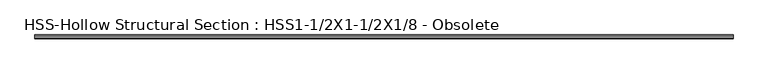
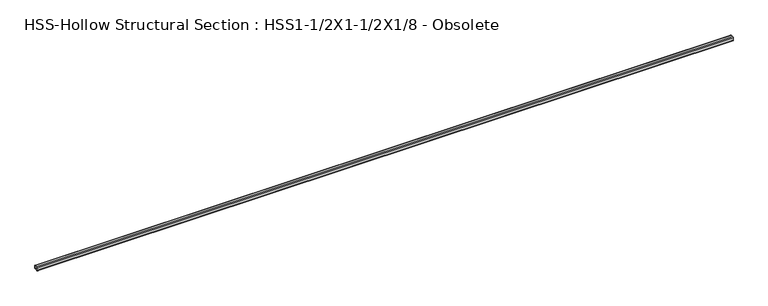
"""IFC4 building model written with IfcOpenShell, lengths in millimetres: beam geometry, HSS-Hollow Structural Section : HSS1-1/2X1-1/2X1/8 - Obsolete."""

from ifc_helpers import new_model, si_unit, point, frame, frame_2d, origin, place, context, project, spatial, polyline, circle_curve, trimmed, segment, composite_curve, outline, extrude, source, transform, mapped, element, save


def hss_hollow_structural_section_hss1_1_2x1_1_2x1_8_obsolete_b716c007(model_context):
    return source(origin(), model_context, "Body", "SweptSolid", [
        extrude(outline(composite_curve([segment(polyline([(19.05, 13.1572), (19.05, -13.1572)]), True, "CONTINUOUS"), segment(trimmed(circle_curve(frame_2d((13.1572, -13.1572)), 5.8928), [point((19.05, -13.1572))], [point((13.1572, -19.05))], False, "CARTESIAN"), True, "CONTINUOUS"), segment(polyline([(13.1572, -19.05), (-13.1572, -19.05)]), True, "CONTINUOUS"), segment(trimmed(circle_curve(frame_2d((-13.1572, -13.1572)), 5.8928), [point((-13.1572, -19.05))], [point((-19.05, -13.1572))], False, "CARTESIAN"), True, "CONTINUOUS"), segment(polyline([(-19.05, -13.1572), (-19.05, 13.1572)]), True, "CONTINUOUS"), segment(trimmed(circle_curve(frame_2d((-13.1572, 13.1572)), 5.8928), [point((-19.05, 13.1572))], [point((-13.1572, 19.05))], False, "CARTESIAN"), True, "CONTINUOUS"), segment(polyline([(-13.1572, 19.05), (13.1572, 19.05)]), True, "CONTINUOUS"), segment(trimmed(circle_curve(frame_2d((13.1572, 13.1572)), 5.8928), [point((13.1572, 19.05))], [point((19.05, 13.1572))], False, "CARTESIAN"), True, "CONTINUOUS")], self_intersect=False), holes=[composite_curve([segment(trimmed(circle_curve(frame_2d((-13.1572, 13.1572)), 2.9464), [point((-13.1572, 16.1036))], [point((-16.1036, 13.1572))], True, "CARTESIAN"), True, "CONTINUOUS"), segment(polyline([(-16.1036, 13.1572), (-16.1036, -13.1572)]), True, "CONTINUOUS"), segment(trimmed(circle_curve(frame_2d((-13.1572, -13.1572)), 2.9464), [point((-16.1036, -13.1572))], [point((-13.1572, -16.1036))], True, "CARTESIAN"), True, "CONTINUOUS"), segment(polyline([(-13.1572, -16.1036), (13.1572, -16.1036)]), True, "CONTINUOUS"), segment(trimmed(circle_curve(frame_2d((13.1572, -13.1572)), 2.9464), [point((13.1572, -16.1036))], [point((16.1036, -13.1572))], True, "CARTESIAN"), True, "CONTINUOUS"), segment(polyline([(16.1036, -13.1572), (16.1036, 13.1572)]), True, "CONTINUOUS"), segment(trimmed(circle_curve(frame_2d((13.1572, 13.1572)), 2.9464), [point((16.1036, 13.1572))], [point((13.1572, 16.1036))], True, "CARTESIAN"), True, "CONTINUOUS"), segment(polyline([(13.1572, 16.1036), (-13.1572, 16.1036)]), True, "CONTINUOUS")], self_intersect=False)]), frame((-3370.2625, 0.0, 0.0), z_axis=(1.0, 0.0, 0.0), x_axis=(0.0, 1.0, 0.0)), (0.0, 0.0, 1.0), 6740.525),
    ])


if __name__ == "__main__":
    model = new_model("IFC4")
    model_context = context("Model", 3, world=origin())
    ifc_project = project(units=[si_unit("LENGTHUNIT", "METRE", prefix="MILLI")], contexts=[model_context])
    site = spatial("IfcSite", under=ifc_project)
    building = spatial("IfcBuilding", under=site)
    placement = place(None, origin())
    hss_hollow_structural_section_hss1_1_2x1_1_2x1_8_obsolete_shape = hss_hollow_structural_section_hss1_1_2x1_1_2x1_8_obsolete_b716c007(model_context)
    element("IfcBeam", 1, ObjectType="HSS-Hollow Structural Section : HSS1-1/2X1-1/2X1/8 - Obsolete", at=placement, inside=building, context=model_context, shape_type="MappedRepresentation", body=[
        mapped(hss_hollow_structural_section_hss1_1_2x1_1_2x1_8_obsolete_shape, transform((0.0, 0.0, 0.0), x_axis=(1.0, 0.0, 0.0), y_axis=(0.0, 1.0, 0.0), z_axis=(0.0, 0.0, 1.0))),
    ])
    save(model, "model.ifc")

# Revit data of these elements
# Type "HSS-Hollow Structural Section : HSS1-1/2X1-1/2X1/8 - Obsolete"
#   Assembly Code = "B10"
#   Shape = "Square"
#   W = 2.19
#   Ht = 0' - 1 1/2"
#   Length [instance default] = 5' - 0"
#   b = 0' - 1 1/2"
#   kr = 0' - 0.232"
#   t = 0' - 0.116"
#   A = 0.00423611 SF
#   Structural Material [instance default] = 1 1/2" X 1 1/2" SPLIT-SEAM SQUARE TUBING (~24" CANTILEVER FROM C.L. OF GLULAM)
# Element 1 (IfcBeam, "HSS-Hollow Structural Section : HSS1-1/2X1-1/2X1/8 - Obsolete")
#   Materials on its faces: "1 1/2\" X 1 1/2\" SPLIT-SEAM SQUARE TUBING (~24\" CANTILEVER FROM C.L. OF GLULAM)"
# Materials
#   "1 1/2\" X 1 1/2\" SPLIT-SEAM SQUARE TUBING (~24\" CANTILEVER FROM C.L. OF GLULAM)": class "Metal", colour RGB 199 199 199, transparency 0, Description = "Carbon steel", Cost = 0
